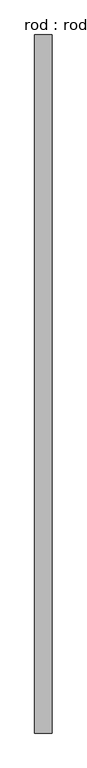
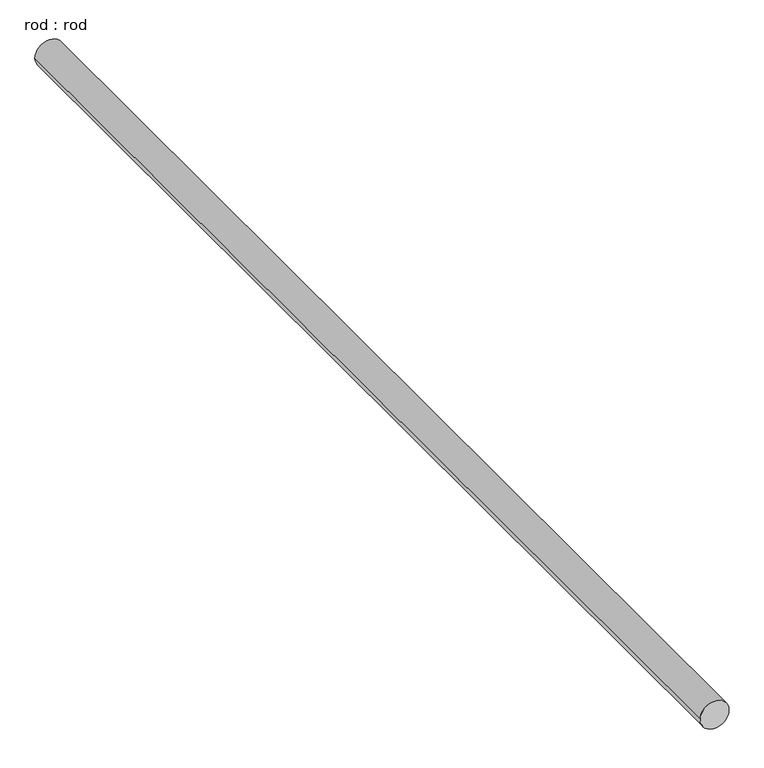
"""IFC4 building model written with IfcOpenShell, lengths in millimetres: proxy geometry, rod : rod."""

from ifc_helpers import new_model, si_unit, point, frame, frame_2d, origin, place, context, project, spatial, circle_curve, trimmed, segment, composite_curve, outline, extrude, source, transform, mapped, element, save


def rod_rod_fd8f4c45(model_context):
    return source(origin(), model_context, "Body", "SweptSolid", [
        extrude(outline(composite_curve([segment(trimmed(circle_curve(frame_2d((0.0108462, 0.0)), 200.0), [point((0.0108462, 200.0))], [point((0.0108462, -200.0))], False, "CARTESIAN"), True, "CONTINUOUS"), segment(trimmed(circle_curve(frame_2d((0.0108462, 0.0)), 200.0), [point((0.0108462, -200.0))], [point((0.0108462, 200.0))], False, "CARTESIAN"), True, "CONTINUOUS")], self_intersect=False)), frame((0.0, -3898.4888295, 0.0), z_axis=(0.0, 1.0, 0.0), x_axis=(0.0, 0.0, 1.0)), (0.0, 0.0, 1.0), 15982.4348896),
    ])


if __name__ == "__main__":
    model = new_model("IFC4")
    model_context = context("Model", 3, world=origin())
    ifc_project = project(units=[si_unit("LENGTHUNIT", "METRE", prefix="MILLI")], contexts=[model_context])
    site = spatial("IfcSite", under=ifc_project)
    building = spatial("IfcBuilding", under=site)
    placement = place(None, origin())
    rod_rod_shape = rod_rod_fd8f4c45(model_context)
    element("IfcBuildingElementProxy", 1, Name="rod : rod", ObjectType="rod : rod", at=placement, inside=building, context=model_context, shape_type="MappedRepresentation", body=[
        mapped(rod_rod_shape, transform((0.0, 0.0, 0.0), x_axis=(1.0, 0.0, 0.0), y_axis=(0.0, 1.0, 0.0), z_axis=(0.0, 0.0, 1.0))),
    ])
    save(model, "model.ifc")

# Revit data of these elements
# Type "rod : rod"
#   Default Elevation = 0
